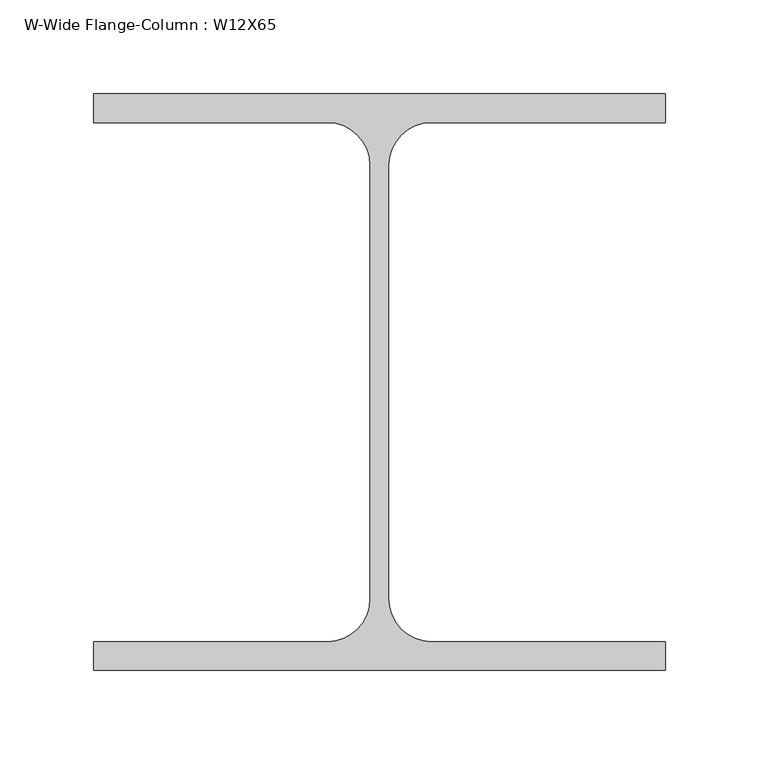
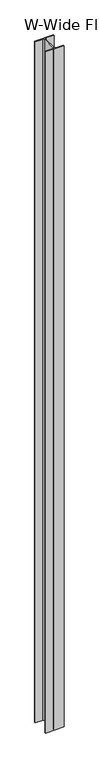
"""IFC4 building model written with IfcOpenShell, lengths in millimetres: column geometry, W-Wide Flange-Column : W12X65."""

from ifc_helpers import new_model, si_unit, point, frame, frame_2d, origin, place, context, project, spatial, polyline, circle_curve, trimmed, segment, composite_curve, outline, extrude, source, transform, mapped, element, save


def w_wide_flange_column_w12x65_f5df1b10(model_context):
    return source(origin(), model_context, "Body", "SweptSolid", [
        extrude(outline(composite_curve([segment(polyline([(152.4, 153.67), (152.4, 138.303), (27.686, 138.303)]), True, "CONTINUOUS"), segment(trimmed(circle_curve(frame_2d((27.686, 115.57)), 22.733), [point((27.686, 138.303))], [point((4.953, 115.57))], True, "CARTESIAN"), True, "CONTINUOUS"), segment(polyline([(4.953, 115.57), (4.953, -115.57)]), True, "CONTINUOUS"), segment(trimmed(circle_curve(frame_2d((27.686, -115.57)), 22.733), [point((4.953, -115.57))], [point((27.686, -138.303))], True, "CARTESIAN"), True, "CONTINUOUS"), segment(polyline([(27.686, -138.303), (152.4, -138.303), (152.4, -153.67), (-152.4, -153.67), (-152.4, -138.303), (-27.686, -138.303)]), True, "CONTINUOUS"), segment(trimmed(circle_curve(frame_2d((-27.686, -115.57)), 22.733), [point((-27.686, -138.303))], [point((-4.953, -115.57))], True, "CARTESIAN"), True, "CONTINUOUS"), segment(polyline([(-4.953, -115.57), (-4.953, 115.57)]), True, "CONTINUOUS"), segment(trimmed(circle_curve(frame_2d((-27.686, 115.57)), 22.733), [point((-4.953, 115.57))], [point((-27.686, 138.303))], True, "CARTESIAN"), True, "CONTINUOUS"), segment(polyline([(-27.686, 138.303), (-152.4, 138.303), (-152.4, 153.67), (152.4, 153.67)]), True, "CONTINUOUS")], self_intersect=False)), frame((0.0, 0.0, 11550.65), z_axis=(0.0, 0.0, 1.0), x_axis=(1.0, 0.0, 0.0)), (0.0, 0.0, 1.0), 11766.55),
    ])


if __name__ == "__main__":
    model = new_model("IFC4")
    model_context = context("Model", 3, world=origin())
    ifc_project = project(units=[si_unit("LENGTHUNIT", "METRE", prefix="MILLI")], contexts=[model_context])
    site = spatial("IfcSite", under=ifc_project)
    building = spatial("IfcBuilding", under=site)
    placement = place(None, origin())
    w_wide_flange_column_w12x65_shape = w_wide_flange_column_w12x65_f5df1b10(model_context)
    element("IfcColumn", 1, ObjectType="W-Wide Flange-Column : W12X65", at=placement, inside=building, context=model_context, shape_type="MappedRepresentation", body=[
        mapped(w_wide_flange_column_w12x65_shape, transform((0.0, 0.0, 0.0), x_axis=(1.0, 0.0, 0.0), y_axis=(0.0, 1.0, 0.0), z_axis=(0.0, 0.0, 1.0))),
    ])
    save(model, "model.ifc")

# Revit data of these elements
# Type "W-Wide Flange-Column : W12X65"
#   Assembly Code = "B10"
#   W = 65
#   bf = 1' - 0"
#   d = 1' - 0.1"
#   k = 0' - 1 1/2"
#   kr = 0' - 0.895"
#   tf = 0' - 0.605"
#   tw = 0' - 0.39"
#   A = 0.132639 SF
#   Structural Material [instance default] = Steel ASTM A992
# Element 1 (IfcColumn, "W-Wide Flange-Column : W12X65")
#   Materials on its faces: "Steel ASTM A992"
# Materials
#   "Steel ASTM A992": class "Metal", colour RGB 199 199 199, transparency 0, Description = "Structural steel 50ksi", Cost = 0
